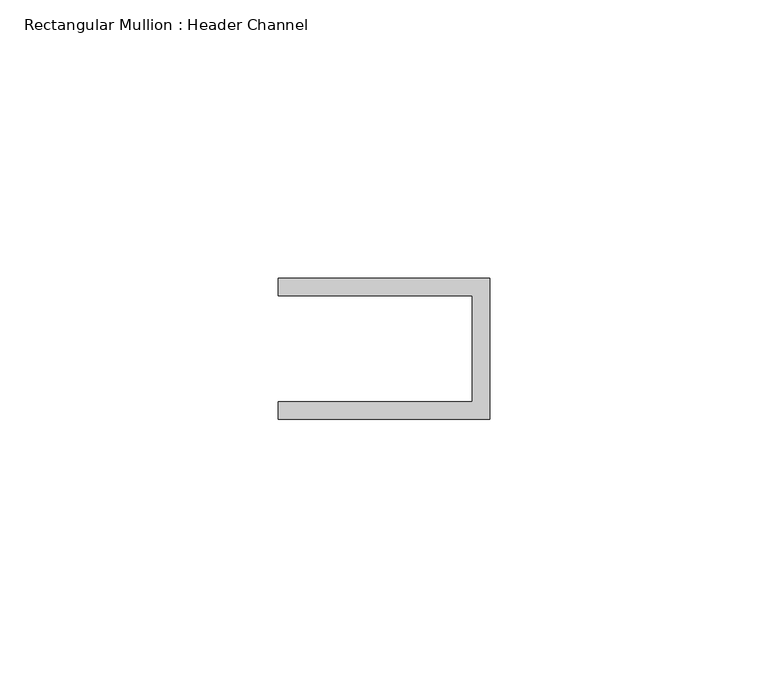
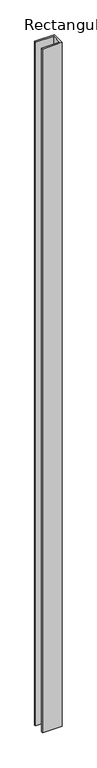
"""IFC4 building model written with IfcOpenShell, lengths in millimetres: member geometry, Rectangular Mullion : Header Channel."""

import ifcopenshell
import ifcopenshell.guid

model = None  # the IFC model being written
_history = None  # IfcOwnerHistory: only IFC2X3 demands one
_inside = {}  # id of a spatial element -> (the spatial element, [elements in it])
_under = {}  # id of a project, library or spatial element -> (it, [spatial elements below it])
_declared = {}  # id of a project -> (the project, [libraries it declares])
_typed = {}  # id of a type object -> (the type object, [elements of that type])
_made_of = {}  # id of a material, layer set ... -> (it, [elements and type objects made of it])


def new_model(schema):
    """Start an empty IFC model of exactly this schema.

    Asked for "IFC4X3", IfcOpenShell would pick the latest addendum, in which some entities
    have other attributes; the version numbers below select the first issue.
    IFC2X3 requires an IfcOwnerHistory on every rooted entity: one is made here for all.
    """
    global model, _history
    if schema == "IFC4X3":
        model = ifcopenshell.file(schema_version=(4, 3, 0, 0))
    else:
        model = ifcopenshell.file(schema=schema)
    _inside.clear()
    _under.clear()
    _declared.clear()
    _typed.clear()
    _made_of.clear()
    _history = None
    if model.schema == "IFC2X3":
        org = make("IfcOrganization", Name="unknown")
        user = make(
            "IfcPersonAndOrganization",
            ThePerson=make("IfcPerson", FamilyName="unknown"),
            TheOrganization=org,
        )
        app = make(
            "IfcApplication",
            ApplicationDeveloper=org,
            Version="unknown",
            ApplicationFullName="unknown",
            ApplicationIdentifier="unknown",
        )
        _history = make(
            "IfcOwnerHistory",
            OwningUser=user,
            OwningApplication=app,
            ChangeAction="ADDED",
            CreationDate=0,
        )
    return model


def make(cls, **values):
    """One entity of the class cls with the attributes given. An attribute that is None is left unset."""
    return model.create_entity(
        cls, **{name: value for name, value in values.items() if value is not None}
    )


def rooted(cls, **values):
    """An entity with a GlobalId (a new one), such as an element, a storey or a relation."""
    return make(cls, GlobalId=ifcopenshell.guid.new(), OwnerHistory=_history, **values)


def si_unit(unit_type, name, prefix=None):
    """IfcSIUnit, for example si_unit("LENGTHUNIT", "METRE", prefix="MILLI")."""
    return make("IfcSIUnit", UnitType=unit_type, Prefix=prefix, Name=name)


def assignment(units):
    """IfcUnitAssignment: the units of a project."""
    return None if units is None else make("IfcUnitAssignment", Units=units)


def point(xyz):
    """IfcCartesianPoint."""
    return None if xyz is None else make("IfcCartesianPoint", Coordinates=xyz)


def direction(xyz):
    """IfcDirection."""
    return None if xyz is None else make("IfcDirection", DirectionRatios=xyz)


def frame(location, z_axis=None, x_axis=None):
    """IfcAxis2Placement3D, a coordinate frame: its origin and axes. An axis left out is left unset."""
    return make(
        "IfcAxis2Placement3D",
        Location=point(location),
        Axis=direction(z_axis),
        RefDirection=direction(x_axis),
    )


def origin():
    """The frame at (0, 0, 0) with its axes left unset."""
    return frame((0.0, 0.0, 0.0))


def place(relative_to, where):
    """IfcLocalPlacement: puts the frame where relative to a parent placement (None: the world)."""
    return make(
        "IfcLocalPlacement", PlacementRelTo=relative_to, RelativePlacement=where
    )


def context(
    kind, dimensions, precision=None, world=None, true_north=None, identifier=None
):
    """IfcGeometricRepresentationContext, for example the 3D "Model" context."""
    return make(
        "IfcGeometricRepresentationContext",
        ContextIdentifier=identifier,
        ContextType=kind,
        CoordinateSpaceDimension=dimensions,
        Precision=precision,
        WorldCoordinateSystem=world,
        TrueNorth=true_north,
    )


def project(units=None, contexts=None):
    """IfcProject with its units and contexts."""
    return rooted(
        "IfcProject",
        Name="project",
        RepresentationContexts=contexts,
        UnitsInContext=assignment(units),
    )


def spatial(cls, under=None, at=None, **own):
    """A site, building, storey or space (cls), placed at a placement, below another one or the project."""
    s = rooted(cls, ObjectPlacement=at, **own)
    if under is not None:
        _under.setdefault(under.id(), (under, []))[1].append(s)
    return s


def polyline(points):
    """IfcPolyline through the points."""
    return make("IfcPolyline", Points=[point(p) for p in points])


def outline(outer, holes=None, kind="AREA"):
    """IfcArbitraryClosedProfileDef: a profile drawn as a closed curve; with holes, ...WithVoids."""
    if holes is None:
        return make("IfcArbitraryClosedProfileDef", ProfileType=kind, OuterCurve=outer)
    return make(
        "IfcArbitraryProfileDefWithVoids",
        ProfileType=kind,
        OuterCurve=outer,
        InnerCurves=holes,
    )


def extrude(swept, where, along, depth):
    """IfcExtrudedAreaSolid: the profile swept, set in the frame where, extruded along a direction by depth."""
    return make(
        "IfcExtrudedAreaSolid",
        SweptArea=swept,
        Position=where,
        ExtrudedDirection=direction(along),
        Depth=depth,
    )


def shape(context_of_items, identifier, shape_type, items):
    """IfcShapeRepresentation: the items that make up one representation, for example the "Body"."""
    return make(
        "IfcShapeRepresentation",
        ContextOfItems=context_of_items,
        RepresentationIdentifier=identifier,
        RepresentationType=shape_type,
        Items=items,
    )


def source(mapping_origin, context_of_items, identifier, shape_type, items):
    """IfcRepresentationMap: a shape defined once, which mapped items show again and again."""
    return make(
        "IfcRepresentationMap",
        MappingOrigin=mapping_origin,
        MappedRepresentation=shape(context_of_items, identifier, shape_type, items),
    )


def transform(
    local_origin,
    x_axis=None,
    y_axis=None,
    z_axis=None,
    scale=None,
    scale2=None,
    scale3=None,
    uniform=True,
):
    """IfcCartesianTransformationOperator3D, or its non-uniform kind. x_axis, y_axis, z_axis: its Axis1, 2, 3."""
    if uniform:
        return make(
            "IfcCartesianTransformationOperator3D",
            Axis1=direction(x_axis),
            Axis2=direction(y_axis),
            LocalOrigin=point(local_origin),
            Scale=scale,
            Axis3=direction(z_axis),
        )
    return make(
        "IfcCartesianTransformationOperator3DnonUniform",
        Axis1=direction(x_axis),
        Axis2=direction(y_axis),
        LocalOrigin=point(local_origin),
        Scale=scale,
        Axis3=direction(z_axis),
        Scale2=scale2,
        Scale3=scale3,
    )


def mapped(mapping_source, mapping_target):
    """IfcMappedItem: shows the shape of a source again, moved by a transform."""
    return make(
        "IfcMappedItem", MappingSource=mapping_source, MappingTarget=mapping_target
    )


def made_of(thing, what):
    """Note that an element or type object is made of a material, layer set ...; save() writes the relation."""
    if what is not None:
        _made_of.setdefault(what.id(), (what, []))[1].append(thing)
    return thing


def element(
    cls,
    number,
    at=None,
    inside=None,
    cuts=None,
    type_object=None,
    material=None,
    context=None,
    identifier="Body",
    shape_type=None,
    held_by="IfcProductDefinitionShape",
    body=None,
    shapes=None,
    **own,
):
    """One element of the class cls, such as IfcWall. Its Tag is "e" and its number.

    at: its placement. inside: the storey or other place that contains it. cuts: it is an
    opening in that element (IfcRelVoidsElement). A single representation is given by context,
    identifier, shape_type and body (its items); several are given by shapes. held_by: the class
    of the entity that holds the representations. save() writes the other relations.
    """
    e = rooted(cls, Tag="e%d" % number, ObjectPlacement=at, **own)
    if body is not None:
        shapes = [shape(context, identifier, shape_type, body)]
    if shapes is not None:
        e.Representation = make(held_by, Representations=shapes)
    if inside is not None:
        _inside.setdefault(inside.id(), (inside, []))[1].append(e)
    if cuts is not None:
        rooted(
            "IfcRelVoidsElement", RelatingBuildingElement=cuts, RelatedOpeningElement=e
        )
    if type_object is not None:
        _typed.setdefault(type_object.id(), (type_object, []))[1].append(e)
    return made_of(e, material)


def aggregate(whole, parts):
    """IfcRelAggregates: a whole, such as a stair, and the parts it consists of."""
    return rooted("IfcRelAggregates", RelatingObject=whole, RelatedObjects=parts)


def save(model, path):
    """Write the relations noted so far, then the file.

    IfcRelAggregates (storeys below a building ...), IfcRelContainedInSpatialStructure (elements
    in a storey), IfcRelDefinesByType, IfcRelAssociatesMaterial and IfcRelDeclares: one each for
    every whole, place, type object, material and project.
    """
    for whole, parts in _under.values():
        aggregate(whole, parts)
    for where, things in _inside.values():
        rooted(
            "IfcRelContainedInSpatialStructure",
            RelatedElements=things,
            RelatingStructure=where,
        )
    for kind, things in _typed.values():
        rooted("IfcRelDefinesByType", RelatedObjects=things, RelatingType=kind)
    for what, things in _made_of.values():
        rooted("IfcRelAssociatesMaterial", RelatedObjects=things, RelatingMaterial=what)
    for by, libraries in _declared.values():
        rooted("IfcRelDeclares", RelatingContext=by, RelatedDefinitions=libraries)
    model.write(path)


def rectangular_mullion_header_channel_0d6f5b44(model_context):
    return source(origin(), model_context, "Body", "SweptSolid", [
        extrude(outline(polyline([(0.0, -12.7), (-38.1, -12.7), (-38.1, -9.525), (-3.175, -9.525), (-3.175, 9.525), (-38.1, 9.525), (-38.1, 12.7), (0.0, 12.7), (0.0, -12.7)])), frame((0.0, 0.0, -1390.6372391), z_axis=(0.0, 0.0, 1.0), x_axis=(1.0, 0.0, 0.0)), (0.0, 0.0, 1.0), 1390.6372391),
    ])


if __name__ == "__main__":
    model = new_model("IFC4")
    model_context = context("Model", 3, world=origin())
    ifc_project = project(units=[si_unit("LENGTHUNIT", "METRE", prefix="MILLI")], contexts=[model_context])
    site = spatial("IfcSite", under=ifc_project)
    building = spatial("IfcBuilding", under=site)
    placement = place(None, origin())
    rectangular_mullion_header_channel_shape = rectangular_mullion_header_channel_0d6f5b44(model_context)
    element("IfcMember", 1, ObjectType="Rectangular Mullion : Header Channel", at=placement, inside=building, context=model_context, shape_type="MappedRepresentation", body=[
        mapped(rectangular_mullion_header_channel_shape, transform((0.0, 0.0, 0.0), x_axis=(1.0, 0.0, 0.0), y_axis=(0.0, 1.0, 0.0), z_axis=(0.0, 0.0, 1.0))),
    ])
    save(model, "model.ifc")

# Revit data of these elements
# Type "Rectangular Mullion : Header Channel"
#   built-in parameter 1007322 = 0.0833333 (stored number, unit not read)
#   built-in parameter 1007321 = -0.03125 (stored number, unit not read)
#   built-in parameter 1007320 = 0.0416667 (stored number, unit not read)
# Element 1 (IfcMember, "Rectangular Mullion : Header Channel")
#   Materials on its faces: "ALUM"
# Materials
#   "ALUM": class "Generic", colour RGB 157 157 157, transparency 0, Cost = 0
